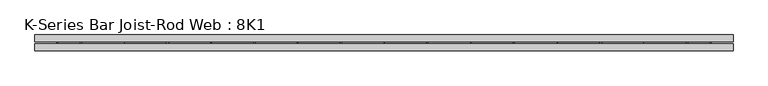
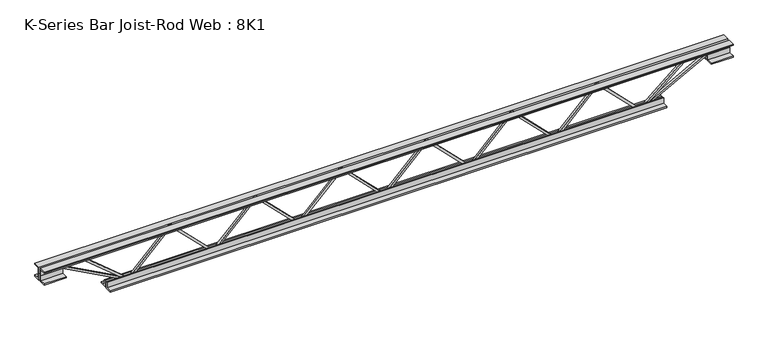
"""IFC4 building model written with IfcOpenShell, lengths in millimetres: beam geometry, K-Series Bar Joist-Rod Web : 8K1."""

from ifc_helpers import new_model, si_unit, frame, origin, place, context, project, spatial, polyline, outline, extrude, source, transform, mapped, element, save


def k_series_bar_joist_rod_web_8k1_218abb50(model_context):
    return source(origin(), model_context, "Body", "SweptSolid", [
        extrude(outline(polyline([(-90.4875, 393.2938636), (-100.0125, 393.2938636), (-100.0125, 398.4430436), (90.4875, 588.7399754), (90.4875, 591.1416154), (-100.0125, 781.4385472), (-100.0125, 786.5877272), (-90.4875, 786.5877272), (-90.4875, 785.3869072), (100.0125, 595.0899754), (100.0125, 584.7916154), (-90.4875, 394.4946836), (-90.4875, 393.2938636)])), frame((0.0, -4.7625, 0.0), z_axis=(0.0, 1.0, 0.0), x_axis=(0.0, 0.0, 1.0)), (0.0, 0.0, 1.0), 9.525),
        extrude(outline(polyline([(-90.4875, 0.0), (-100.0125, 0.0), (-100.0125, 5.14918), (90.4875, 195.4461118), (90.4875, 197.8477518), (-100.0125, 388.1446836), (-100.0125, 393.2938636), (-90.4875, 393.2938636), (-90.4875, 392.0930436), (100.0125, 201.7961118), (100.0125, 191.4977518), (-90.4875, 1.20082), (-90.4875, 0.0)])), frame((0.0, -4.7625, 0.0), z_axis=(0.0, 1.0, 0.0), x_axis=(0.0, 0.0, 1.0)), (0.0, 0.0, 1.0), 9.525),
        extrude(outline(polyline([(-90.4875, -393.2938636), (-100.0125, -393.2938636), (-100.0125, -388.1446836), (90.4875, -197.8477518), (90.4875, -195.4461118), (-100.0125, -5.14918), (-100.0125, 0.0), (-90.4875, 0.0), (-90.4875, -1.20082), (100.0125, -191.4977518), (100.0125, -201.7961118), (-90.4875, -392.0930436), (-90.4875, -393.2938636)])), frame((0.0, -4.7625, 0.0), z_axis=(0.0, 1.0, 0.0), x_axis=(0.0, 0.0, 1.0)), (0.0, 0.0, 1.0), 9.525),
        extrude(outline(polyline([(-90.4875, -786.5877272), (-100.0125, -786.5877272), (-100.0125, -781.4385472), (90.4875, -591.1416154), (90.4875, -588.7399754), (-100.0125, -398.4430436), (-100.0125, -393.2938636), (-90.4875, -393.2938636), (-90.4875, -394.4946836), (100.0125, -584.7916154), (100.0125, -595.0899754), (-90.4875, -785.3869072), (-90.4875, -786.5877272)])), frame((0.0, -4.7625, 0.0), z_axis=(0.0, 1.0, 0.0), x_axis=(0.0, 0.0, 1.0)), (0.0, 0.0, 1.0), 9.525),
        extrude(outline(polyline([(-90.4875, 786.5877272), (-100.0125, 786.5877272), (-100.0125, 791.7369072), (90.4875, 982.033839), (90.4875, 984.435479), (-100.0125, 1174.7324108), (-100.0125, 1179.8815908), (-90.4875, 1179.8815908), (-90.4875, 1178.6807708), (100.0125, 988.383839), (100.0125, 978.085479), (-90.4875, 787.7885472), (-90.4875, 786.5877272)])), frame((0.0, -4.7625, 0.0), z_axis=(0.0, 1.0, 0.0), x_axis=(0.0, 0.0, 1.0)), (0.0, 0.0, 1.0), 9.525),
        extrude(outline(polyline([(-90.4875, -1179.8815908), (-100.0125, -1179.8815908), (-100.0125, -1174.7324108), (90.4875, -984.435479), (90.4875, -982.033839), (-100.0125, -791.7369072), (-100.0125, -786.5877272), (-90.4875, -786.5877272), (-90.4875, -787.7885472), (100.0125, -978.085479), (100.0125, -988.383839), (-90.4875, -1178.6807708), (-90.4875, -1179.8815908)])), frame((0.0, -4.7625, 0.0), z_axis=(0.0, 1.0, 0.0), x_axis=(0.0, 0.0, 1.0)), (0.0, 0.0, 1.0), 9.525),
        extrude(outline(polyline([(4.7625, 101.6), (36.5125, 101.6), (36.5125, 95.25), (11.1125, 95.25), (11.1125, 69.85), (4.7625, 69.85), (4.7625, 101.6)])), frame((-1586.2815908, 0.0, 0.0), z_axis=(1.0, 0.0, 0.0), x_axis=(0.0, 1.0, 0.0)), (0.0, 0.0, 1.0), 3172.5631816),
        extrude(outline(polyline([(-4.7625, 101.6), (-4.7625, 69.85), (-11.1125, 69.85), (-11.1125, 95.25), (-36.5125, 95.25), (-36.5125, 101.6), (-4.7625, 101.6)])), frame((-1586.2815908, 0.0, 0.0), z_axis=(1.0, 0.0, 0.0), x_axis=(0.0, 1.0, 0.0)), (0.0, 0.0, 1.0), 3172.5631816),
        extrude(outline(polyline([(-4.7625, 38.1), (-36.5125, 38.1), (-36.5125, 44.45), (-11.1125, 44.45), (-11.1125, 69.85), (-4.7625, 69.85), (-4.7625, 38.1)])), frame((-1586.2815908, 0.0, 0.0), z_axis=(1.0, 0.0, 0.0), x_axis=(0.0, 1.0, 0.0)), (0.0, 0.0, 1.0), 101.6),
        extrude(outline(polyline([(36.5125, 38.1), (4.7625, 38.1), (4.7625, 69.85), (11.1125, 69.85), (11.1125, 44.45), (36.5125, 44.45), (36.5125, 38.1)])), frame((-1586.2815908, 0.0, 0.0), z_axis=(1.0, 0.0, 0.0), x_axis=(0.0, 1.0, 0.0)), (0.0, 0.0, 1.0), 101.6),
        extrude(outline(polyline([(4.7625, 38.1), (4.7625, 69.85), (11.1125, 69.85), (11.1125, 44.45), (36.5125, 44.45), (36.5125, 38.1), (4.7625, 38.1)])), frame((1484.6815908, 0.0, 0.0), z_axis=(1.0, 0.0, 0.0), x_axis=(0.0, 1.0, 0.0)), (0.0, 0.0, 1.0), 101.6),
        extrude(outline(polyline([(-4.7625, 38.1), (-36.5125, 38.1), (-36.5125, 44.45), (-11.1125, 44.45), (-11.1125, 69.85), (-4.7625, 69.85), (-4.7625, 38.1)])), frame((1484.6815908, 0.0, 0.0), z_axis=(1.0, 0.0, 0.0), x_axis=(0.0, 1.0, 0.0)), (0.0, 0.0, 1.0), 101.6),
        extrude(outline(polyline([(4.7625, -101.6), (4.7625, -69.85), (11.1125, -69.85), (11.1125, -95.25), (36.5125, -95.25), (36.5125, -101.6), (4.7625, -101.6)])), frame((-1281.4815908, 0.0, 0.0), z_axis=(1.0, 0.0, 0.0), x_axis=(0.0, 1.0, 0.0)), (0.0, 0.0, 1.0), 2562.9631816),
        extrude(outline(polyline([(-4.7625, -101.6), (-36.5125, -101.6), (-36.5125, -95.25), (-11.1125, -95.25), (-11.1125, -69.85), (-4.7625, -69.85), (-4.7625, -101.6)])), frame((-1281.4815908, 0.0, 0.0), z_axis=(1.0, 0.0, 0.0), x_axis=(0.0, 1.0, 0.0)), (0.0, 0.0, 1.0), 2562.9631816),
        extrude(outline(polyline([(0.0, -9.525), (0.0, 0.0), (346.6425392, 0.0), (346.6425392, -9.525), (0.0, -9.525)])), frame((-1486.9498893, 4.7625, 65.662372), z_axis=(0.4762831485400801, 0.0, 0.8792919665371384), x_axis=(0.8792919665371384, 0.0, -0.4762831485400801)), (0.0, 0.0, 1.0), 9.525),
        extrude(outline(polyline([(0.0, -9.525), (0.0, 0.0), (256.7645337, 0.0), (256.7645337, -9.525), (0.0, -9.525)])), frame((-1379.5908176, 4.7625, 66.2025686), z_axis=(0.6430015765679582, 0.0, 0.7658648526542527), x_axis=(0.7658648526542527, 0.0, -0.6430015765679582)), (0.0, 0.0, 1.0), 9.525),
        extrude(outline(polyline([(0.0, -9.525), (0.0, 0.0), (346.6425392, 0.0), (346.6425392, -9.525), (0.0, -9.525)])), frame((1486.9498893, -4.7625, 65.662372), z_axis=(-0.4762831485400414, 0.0, 0.8792919665371594), x_axis=(-0.8792919665371594, 0.0, -0.4762831485400414)), (0.0, 0.0, 1.0), 9.525),
        extrude(outline(polyline([(0.0, -9.525), (0.0, 0.0), (256.7645337, 0.0), (256.7645337, -9.525), (0.0, -9.525)])), frame((1379.5908176, -4.7625, 66.2025686), z_axis=(-0.6430015765679298, 0.0, 0.7658648526542767), x_axis=(-0.7658648526542767, 0.0, -0.6430015765679298)), (0.0, 0.0, 1.0), 9.525),
    ])


if __name__ == "__main__":
    model = new_model("IFC4")
    model_context = context("Model", 3, world=origin())
    ifc_project = project(units=[si_unit("LENGTHUNIT", "METRE", prefix="MILLI")], contexts=[model_context])
    site = spatial("IfcSite", under=ifc_project)
    building = spatial("IfcBuilding", under=site)
    placement = place(None, origin())
    k_series_bar_joist_rod_web_8k1_shape = k_series_bar_joist_rod_web_8k1_218abb50(model_context)
    element("IfcBeam", 1, ObjectType="K-Series Bar Joist-Rod Web : 8K1", at=placement, inside=building, context=model_context, shape_type="MappedRepresentation", body=[
        mapped(k_series_bar_joist_rod_web_8k1_shape, transform((0.0, 0.0, 0.0), x_axis=(1.0, 0.0, 0.0), y_axis=(0.0, 1.0, 0.0), z_axis=(0.0, 0.0, 1.0))),
    ])
    save(model, "model.ifc")

# Revit data of these elements
# Type "K-Series Bar Joist-Rod Web : 8K1"
#   Assembly Code = "B1010350"
#   Wt = 5.1
#   Web Thickness = 0' - 0 3/8"
#   Start Offset [instance default] = 0' - 0"
#   Start Extension [instance default] = 0' - 0"
#   Seat Length = 0' - 4"
#   Seat Depth = 0' - 2 1/2"
#   PanelArrayLength [instance default] = 21' - 4"
#   Panel [instance default] = 1' - 4"
#   End Offset [instance default] = 0' - 0"
#   End Extension [instance default] = 0' - 0"
#   End Panel = 1' - 4"
#   Cord Leg = 0' - 1 1/4"
#   Chord Thickness = 0' - 0 1/4"
#   Length [instance default] = 24' - 0"
#   Depth = 0' - 8"
#   PanelArrayNum [instance default] = 16
#   Rendering Material = none
# Element 1 (IfcBeam, "K-Series Bar Joist-Rod Web : 8K1")
#   PanelArrayLength = 7' - 8.90406"
#   Panel = 1' - 3.48401"
#   PanelArrayNum = 6
